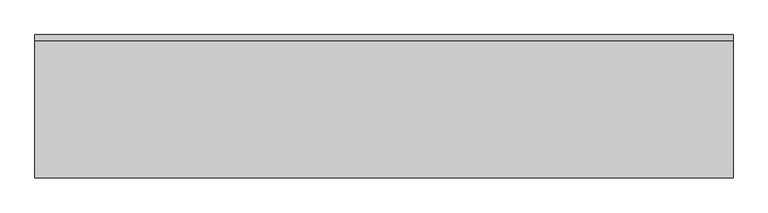
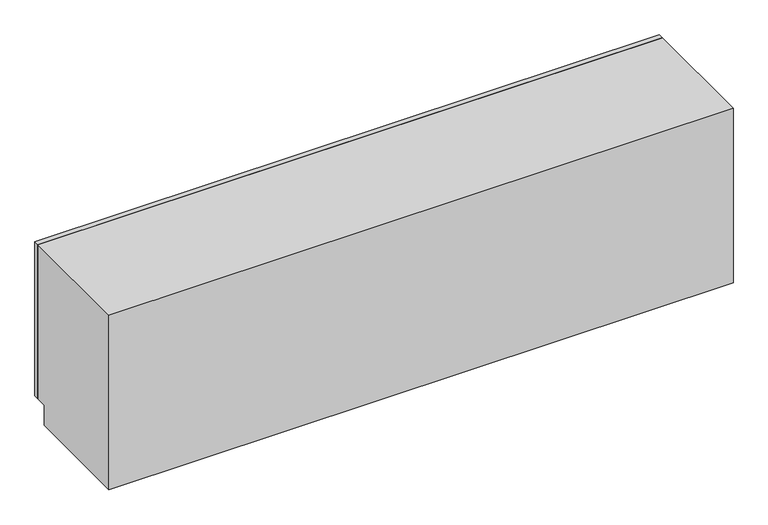
"""IFC4 building model written with IfcOpenShell, lengths in millimetres: furniture geometry, OD_CW_Base Cabinet : OD_CW_Base Cabinet."""

from ifc_helpers import new_model, si_unit, frame, origin, place, context, project, spatial, polyline, outline, extrude, source, transform, mapped, element, save


def furniture_ec971a78(model_context):
    return source(origin(), model_context, "Body", "SweptSolid", [
        extrude(outline(polyline([(18.7377049, -25.4), (18.7377049, 0.0), (2984.1877049, 0.0), (2984.1877049, -25.4), (18.7377049, -25.4)])), frame((0.0, 0.0, 101.6), z_axis=(0.0, 0.0, 1.0), x_axis=(1.0, 0.0, 0.0)), (0.0, 0.0, 1.0), 774.7),
        extrude(outline(polyline([(-25.4, 876.3), (-25.4, 101.6), (-76.2, 101.6), (-76.2, 0.0), (-609.6, 0.0), (-609.6, 876.3), (-25.4, 876.3)])), frame((18.7377049, 0.0, 0.0), z_axis=(1.0, 0.0, 0.0), x_axis=(0.0, 1.0, 0.0)), (0.0, 0.0, 1.0), 2965.45),
    ])


if __name__ == "__main__":
    model = new_model("IFC4")
    model_context = context("Model", 3, world=origin())
    ifc_project = project(units=[si_unit("LENGTHUNIT", "METRE", prefix="MILLI")], contexts=[model_context])
    site = spatial("IfcSite", under=ifc_project)
    building = spatial("IfcBuilding", under=site)
    placement = place(None, origin())
    furniture_shape = furniture_ec971a78(model_context)
    element("IfcFurniture", 1, ObjectType="OD_CW_Base Cabinet : OD_CW_Base Cabinet", at=placement, inside=building, context=model_context, shape_type="MappedRepresentation", body=[
        mapped(furniture_shape, transform((0.0, 0.0, 0.0), x_axis=(1.0, 0.0, 0.0), y_axis=(0.0, 1.0, 0.0), z_axis=(0.0, 0.0, 1.0))),
    ])
    save(model, "model.ifc")

# Revit data of these elements
# Type "OD_CW_Base Cabinet : OD_CW_Base Cabinet"
#   OD_CW_Width [instance default] = 2' - 10"
#   OD_CW_Length [instance default] = 8' - 0"
#   OD_CW_Height [instance default] = 2' - 3"
#   Depth = 2' - 0"
#   Height = 3' - 0"
#   Width = 4' - 0"
#   OD_CW_Material_Front Panel [instance default] = none
#   OD_CW_Material_Body [instance default] = none
# Element 1 (IfcFurniture, "OD_CW_Base Cabinet : OD_CW_Base Cabinet")
#   OD_CW_Width = 2' - 0"
#   OD_CW_Length = 9' - 8 3/4"
#   OD_CW_Height = 2' - 10 1/2"
#   Materials on its faces: "casework"
# Materials
#   "casework": class "Generic", colour RGB 229 229 229, transparency 0, Cost = 0
